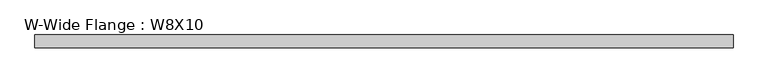
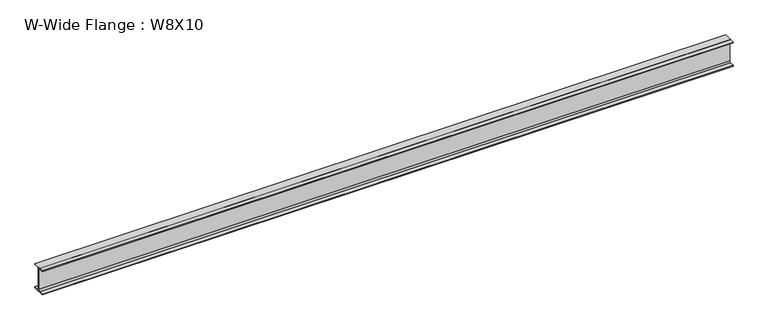
"""IFC4 building model written with IfcOpenShell, lengths in millimetres: beam geometry, W-Wide Flange : W8X10."""

from ifc_helpers import new_model, si_unit, point, frame, frame_2d, origin, place, context, project, spatial, polyline, circle_curve, trimmed, segment, composite_curve, outline, extrude, source, transform, mapped, element, save


def w_wide_flange_w8x10_22581100(model_context):
    return source(origin(), model_context, "Body", "SweptSolid", [
        extrude(outline(composite_curve([segment(polyline([(50.038, -94.996), (50.038, -100.203), (-50.038, -100.203), (-50.038, -94.996), (-14.4145, -94.996)]), True, "CONTINUOUS"), segment(trimmed(circle_curve(frame_2d((-14.4145, -82.7405)), 12.2555), [point((-14.4145, -94.996))], [point((-2.159, -82.7405))], True, "CARTESIAN"), True, "CONTINUOUS"), segment(polyline([(-2.159, -82.7405), (-2.159, 82.7405)]), True, "CONTINUOUS"), segment(trimmed(circle_curve(frame_2d((-14.4145, 82.7405)), 12.2555), [point((-2.159, 82.7405))], [point((-14.4145, 94.996))], True, "CARTESIAN"), True, "CONTINUOUS"), segment(polyline([(-14.4145, 94.996), (-50.038, 94.996), (-50.038, 100.203), (50.038, 100.203), (50.038, 94.996), (14.4145, 94.996)]), True, "CONTINUOUS"), segment(trimmed(circle_curve(frame_2d((14.4145, 82.7405)), 12.2555), [point((14.4145, 94.996))], [point((2.159, 82.7405))], True, "CARTESIAN"), True, "CONTINUOUS"), segment(polyline([(2.159, 82.7405), (2.159, -82.7405)]), True, "CONTINUOUS"), segment(trimmed(circle_curve(frame_2d((14.4145, -82.7405)), 12.2555), [point((2.159, -82.7405))], [point((14.4145, -94.996))], True, "CARTESIAN"), True, "CONTINUOUS"), segment(polyline([(14.4145, -94.996), (50.038, -94.996)]), True, "CONTINUOUS")], self_intersect=False)), frame((-2744.7378906, 0.0, 0.0), z_axis=(1.0, 0.0, 0.0), x_axis=(0.0, 1.0, 0.0)), (0.0, 0.0, 1.0), 5476.5713906),
    ])


if __name__ == "__main__":
    model = new_model("IFC4")
    model_context = context("Model", 3, world=origin())
    ifc_project = project(units=[si_unit("LENGTHUNIT", "METRE", prefix="MILLI")], contexts=[model_context])
    site = spatial("IfcSite", under=ifc_project)
    building = spatial("IfcBuilding", under=site)
    placement = place(None, origin())
    w_wide_flange_w8x10_shape = w_wide_flange_w8x10_22581100(model_context)
    element("IfcBeam", 1, ObjectType="W-Wide Flange : W8X10", at=placement, inside=building, context=model_context, shape_type="MappedRepresentation", body=[
        mapped(w_wide_flange_w8x10_shape, transform((0.0, 0.0, 0.0), x_axis=(1.0, 0.0, 0.0), y_axis=(0.0, 1.0, 0.0), z_axis=(0.0, 0.0, 1.0))),
    ])
    save(model, "model.ifc")

# Revit data of these elements
# Type "W-Wide Flange : W8X10"
#   Assembly Code = "B10"
#   W = 10
#   Length [instance default] = 1524 mm
#   bf = 100.076 mm
#   d = 200.406 mm
#   k = 17.463 mm
#   k2 = 12.255 mm
#   tf = 5.207 mm
#   tw = 4.318 mm
#   A = 0.00190967 m²
#   Structural Material [instance default] = Steel ASTM A992
# Element 1 (IfcBeam, "W-Wide Flange : W8X10")
#   Structural Material = Aluminum, Anodized Red
#   Materials on its faces: "Aluminum, Anodized Red"
# Materials
#   "Steel ASTM A992": class "Metal", colour RGB 128 0 0, transparency 0, Description = "Structural steel 50ksi", Cost = 0
#   "Aluminum, Anodized Red": class "Metal", colour RGB 120 120 120, transparency 0, Description = "Anodized aluminum, red", Cost = 0
